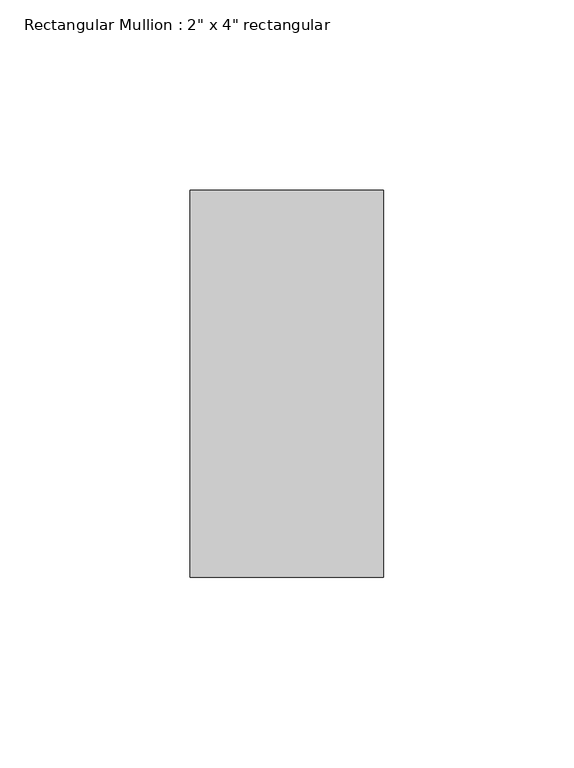
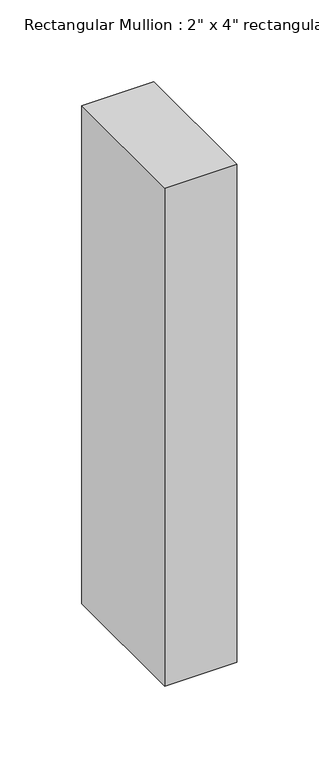
"""IFC4 building model written with IfcOpenShell, lengths in millimetres: member geometry."""

from ifc_helpers import new_model, si_unit, frame, origin, place, context, project, spatial, polyline, outline, extrude, source, transform, mapped, element, save


def member_28c55b95(model_context):
    return source(origin(), model_context, "Body", "SweptSolid", [
        extrude(outline(polyline([(0.0, 50.8), (0.0, -50.8), (-50.8, -50.8), (-50.8, 50.8), (0.0, 50.8)])), frame((0.0, 0.0, -371.9285714), z_axis=(0.0, 0.0, 1.0), x_axis=(1.0, 0.0, 0.0)), (0.0, 0.0, 1.0), 371.9285714),
    ])


if __name__ == "__main__":
    model = new_model("IFC4")
    model_context = context("Model", 3, world=origin())
    ifc_project = project(units=[si_unit("LENGTHUNIT", "METRE", prefix="MILLI")], contexts=[model_context])
    site = spatial("IfcSite", under=ifc_project)
    building = spatial("IfcBuilding", under=site)
    placement = place(None, origin())
    member_shape = member_28c55b95(model_context)
    element("IfcMember", 1, ObjectType="Rectangular Mullion : 2\" x 4\" rectangular", at=placement, inside=building, context=model_context, shape_type="MappedRepresentation", body=[
        mapped(member_shape, transform((0.0, 0.0, 0.0), x_axis=(1.0, 0.0, 0.0), y_axis=(0.0, 1.0, 0.0), z_axis=(0.0, 0.0, 1.0))),
    ])
    save(model, "model.ifc")

# Revit data of these elements
# Type "Rectangular Mullion : 2\" x 4\" rectangular"
#   built-in parameter 1007304 = 0.333333 (stored number, unit not read)
#   built-in parameter 1007301 = 0.0833333 (stored number, unit not read)
#   built-in parameter 1007300 = 0.0833333 (stored number, unit not read)
